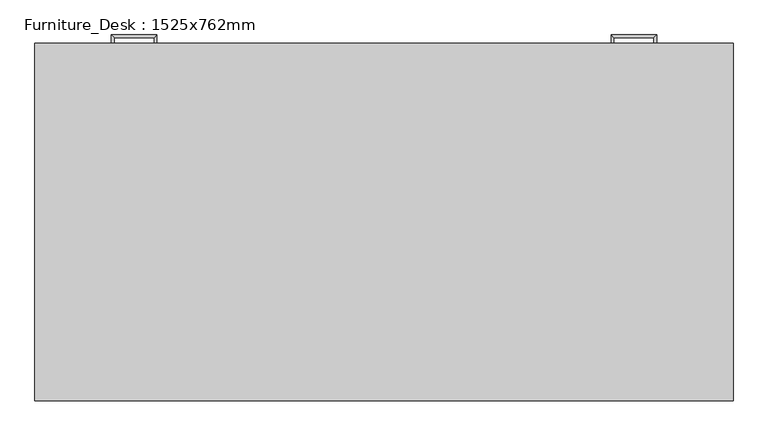
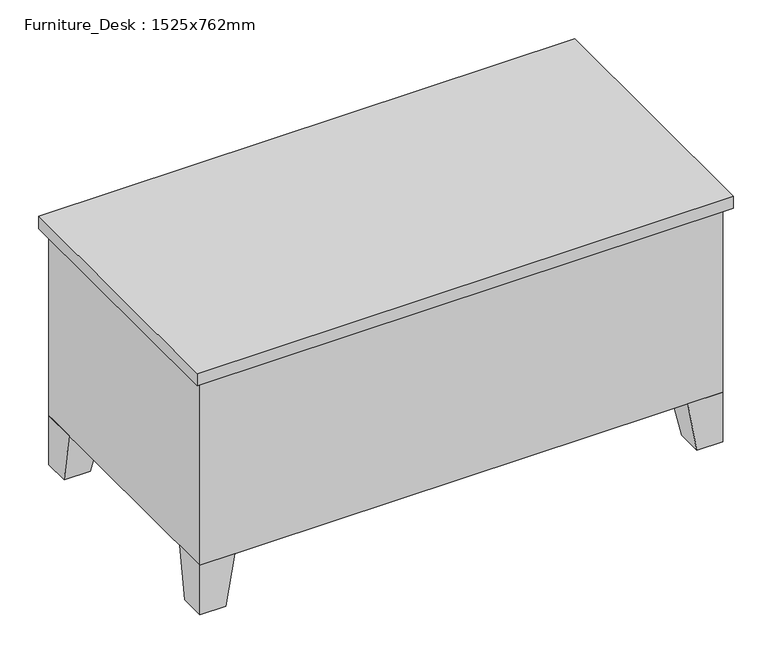
"""IFC4 building model written with IfcOpenShell, lengths in millimetres: furniture geometry, Furniture_Desk : 1525x762mm."""

import ifcopenshell
import ifcopenshell.guid

model = None  # the IFC model being written
_history = None  # IfcOwnerHistory: only IFC2X3 demands one
_inside = {}  # id of a spatial element -> (the spatial element, [elements in it])
_under = {}  # id of a project, library or spatial element -> (it, [spatial elements below it])
_declared = {}  # id of a project -> (the project, [libraries it declares])
_typed = {}  # id of a type object -> (the type object, [elements of that type])
_made_of = {}  # id of a material, layer set ... -> (it, [elements and type objects made of it])


def new_model(schema):
    """Start an empty IFC model of exactly this schema.

    Asked for "IFC4X3", IfcOpenShell would pick the latest addendum, in which some entities
    have other attributes; the version numbers below select the first issue.
    IFC2X3 requires an IfcOwnerHistory on every rooted entity: one is made here for all.
    """
    global model, _history
    if schema == "IFC4X3":
        model = ifcopenshell.file(schema_version=(4, 3, 0, 0))
    else:
        model = ifcopenshell.file(schema=schema)
    _inside.clear()
    _under.clear()
    _declared.clear()
    _typed.clear()
    _made_of.clear()
    _history = None
    if model.schema == "IFC2X3":
        org = make("IfcOrganization", Name="unknown")
        user = make(
            "IfcPersonAndOrganization",
            ThePerson=make("IfcPerson", FamilyName="unknown"),
            TheOrganization=org,
        )
        app = make(
            "IfcApplication",
            ApplicationDeveloper=org,
            Version="unknown",
            ApplicationFullName="unknown",
            ApplicationIdentifier="unknown",
        )
        _history = make(
            "IfcOwnerHistory",
            OwningUser=user,
            OwningApplication=app,
            ChangeAction="ADDED",
            CreationDate=0,
        )
    return model


def make(cls, **values):
    """One entity of the class cls with the attributes given. An attribute that is None is left unset."""
    return model.create_entity(
        cls, **{name: value for name, value in values.items() if value is not None}
    )


def rooted(cls, **values):
    """An entity with a GlobalId (a new one), such as an element, a storey or a relation."""
    return make(cls, GlobalId=ifcopenshell.guid.new(), OwnerHistory=_history, **values)


def si_unit(unit_type, name, prefix=None):
    """IfcSIUnit, for example si_unit("LENGTHUNIT", "METRE", prefix="MILLI")."""
    return make("IfcSIUnit", UnitType=unit_type, Prefix=prefix, Name=name)


def assignment(units):
    """IfcUnitAssignment: the units of a project."""
    return None if units is None else make("IfcUnitAssignment", Units=units)


def point(xyz):
    """IfcCartesianPoint."""
    return None if xyz is None else make("IfcCartesianPoint", Coordinates=xyz)


def direction(xyz):
    """IfcDirection."""
    return None if xyz is None else make("IfcDirection", DirectionRatios=xyz)


def frame(location, z_axis=None, x_axis=None):
    """IfcAxis2Placement3D, a coordinate frame: its origin and axes. An axis left out is left unset."""
    return make(
        "IfcAxis2Placement3D",
        Location=point(location),
        Axis=direction(z_axis),
        RefDirection=direction(x_axis),
    )


def origin():
    """The frame at (0, 0, 0) with its axes left unset."""
    return frame((0.0, 0.0, 0.0))


def place(relative_to, where):
    """IfcLocalPlacement: puts the frame where relative to a parent placement (None: the world)."""
    return make(
        "IfcLocalPlacement", PlacementRelTo=relative_to, RelativePlacement=where
    )


def context(
    kind, dimensions, precision=None, world=None, true_north=None, identifier=None
):
    """IfcGeometricRepresentationContext, for example the 3D "Model" context."""
    return make(
        "IfcGeometricRepresentationContext",
        ContextIdentifier=identifier,
        ContextType=kind,
        CoordinateSpaceDimension=dimensions,
        Precision=precision,
        WorldCoordinateSystem=world,
        TrueNorth=true_north,
    )


def project(units=None, contexts=None):
    """IfcProject with its units and contexts."""
    return rooted(
        "IfcProject",
        Name="project",
        RepresentationContexts=contexts,
        UnitsInContext=assignment(units),
    )


def spatial(cls, under=None, at=None, **own):
    """A site, building, storey or space (cls), placed at a placement, below another one or the project."""
    s = rooted(cls, ObjectPlacement=at, **own)
    if under is not None:
        _under.setdefault(under.id(), (under, []))[1].append(s)
    return s


def polyline(points):
    """IfcPolyline through the points."""
    return make("IfcPolyline", Points=[point(p) for p in points])


def outline(outer, holes=None, kind="AREA"):
    """IfcArbitraryClosedProfileDef: a profile drawn as a closed curve; with holes, ...WithVoids."""
    if holes is None:
        return make("IfcArbitraryClosedProfileDef", ProfileType=kind, OuterCurve=outer)
    return make(
        "IfcArbitraryProfileDefWithVoids",
        ProfileType=kind,
        OuterCurve=outer,
        InnerCurves=holes,
    )


def extrude(swept, where, along, depth):
    """IfcExtrudedAreaSolid: the profile swept, set in the frame where, extruded along a direction by depth."""
    return make(
        "IfcExtrudedAreaSolid",
        SweptArea=swept,
        Position=where,
        ExtrudedDirection=direction(along),
        Depth=depth,
    )


def faces_of(points, faces, orient=None, outer=None):
    """IfcFace entities. A face is a list of loops; a loop is a list of indices into points, from 0.

    orient and outer hold one flag for each loop. By default every Orientation is true, the
    first loop of a face is its IfcFaceOuterBound and the others are IfcFaceBound.
    """
    made = []
    for i, loops in enumerate(faces):
        bounds = []
        for j, loop in enumerate(loops):
            is_outer = j == 0 if outer is None else outer[i][j]
            bounds.append(
                make(
                    "IfcFaceOuterBound" if is_outer else "IfcFaceBound",
                    Bound=make("IfcPolyLoop", Polygon=[points[k] for k in loop]),
                    Orientation=True if orient is None else orient[i][j],
                )
            )
        made.append(make("IfcFace", Bounds=bounds))
    return made


def faceted_brep(points, faces, orient=None, outer=None, voids=None):
    """IfcFacetedBrep: a solid bounded by flat faces; with voids (closed shells), ...WithVoids."""
    shared = [point(p) for p in points]
    hull = make("IfcClosedShell", CfsFaces=faces_of(shared, faces, orient, outer))
    if voids is None:
        return make("IfcFacetedBrep", Outer=hull)
    return make(
        "IfcFacetedBrepWithVoids",
        Outer=hull,
        Voids=[
            make(cls, CfsFaces=faces_of(shared, fs, o, b)) for cls, fs, o, b in voids
        ],
    )


def shape(context_of_items, identifier, shape_type, items):
    """IfcShapeRepresentation: the items that make up one representation, for example the "Body"."""
    return make(
        "IfcShapeRepresentation",
        ContextOfItems=context_of_items,
        RepresentationIdentifier=identifier,
        RepresentationType=shape_type,
        Items=items,
    )


def source(mapping_origin, context_of_items, identifier, shape_type, items):
    """IfcRepresentationMap: a shape defined once, which mapped items show again and again."""
    return make(
        "IfcRepresentationMap",
        MappingOrigin=mapping_origin,
        MappedRepresentation=shape(context_of_items, identifier, shape_type, items),
    )


def transform(
    local_origin,
    x_axis=None,
    y_axis=None,
    z_axis=None,
    scale=None,
    scale2=None,
    scale3=None,
    uniform=True,
):
    """IfcCartesianTransformationOperator3D, or its non-uniform kind. x_axis, y_axis, z_axis: its Axis1, 2, 3."""
    if uniform:
        return make(
            "IfcCartesianTransformationOperator3D",
            Axis1=direction(x_axis),
            Axis2=direction(y_axis),
            LocalOrigin=point(local_origin),
            Scale=scale,
            Axis3=direction(z_axis),
        )
    return make(
        "IfcCartesianTransformationOperator3DnonUniform",
        Axis1=direction(x_axis),
        Axis2=direction(y_axis),
        LocalOrigin=point(local_origin),
        Scale=scale,
        Axis3=direction(z_axis),
        Scale2=scale2,
        Scale3=scale3,
    )


def mapped(mapping_source, mapping_target):
    """IfcMappedItem: shows the shape of a source again, moved by a transform."""
    return make(
        "IfcMappedItem", MappingSource=mapping_source, MappingTarget=mapping_target
    )


def made_of(thing, what):
    """Note that an element or type object is made of a material, layer set ...; save() writes the relation."""
    if what is not None:
        _made_of.setdefault(what.id(), (what, []))[1].append(thing)
    return thing


def element(
    cls,
    number,
    at=None,
    inside=None,
    cuts=None,
    type_object=None,
    material=None,
    context=None,
    identifier="Body",
    shape_type=None,
    held_by="IfcProductDefinitionShape",
    body=None,
    shapes=None,
    **own,
):
    """One element of the class cls, such as IfcWall. Its Tag is "e" and its number.

    at: its placement. inside: the storey or other place that contains it. cuts: it is an
    opening in that element (IfcRelVoidsElement). A single representation is given by context,
    identifier, shape_type and body (its items); several are given by shapes. held_by: the class
    of the entity that holds the representations. save() writes the other relations.
    """
    e = rooted(cls, Tag="e%d" % number, ObjectPlacement=at, **own)
    if body is not None:
        shapes = [shape(context, identifier, shape_type, body)]
    if shapes is not None:
        e.Representation = make(held_by, Representations=shapes)
    if inside is not None:
        _inside.setdefault(inside.id(), (inside, []))[1].append(e)
    if cuts is not None:
        rooted(
            "IfcRelVoidsElement", RelatingBuildingElement=cuts, RelatedOpeningElement=e
        )
    if type_object is not None:
        _typed.setdefault(type_object.id(), (type_object, []))[1].append(e)
    return made_of(e, material)


def aggregate(whole, parts):
    """IfcRelAggregates: a whole, such as a stair, and the parts it consists of."""
    return rooted("IfcRelAggregates", RelatingObject=whole, RelatedObjects=parts)


def save(model, path):
    """Write the relations noted so far, then the file.

    IfcRelAggregates (storeys below a building ...), IfcRelContainedInSpatialStructure (elements
    in a storey), IfcRelDefinesByType, IfcRelAssociatesMaterial and IfcRelDeclares: one each for
    every whole, place, type object, material and project.
    """
    for whole, parts in _under.values():
        aggregate(whole, parts)
    for where, things in _inside.values():
        rooted(
            "IfcRelContainedInSpatialStructure",
            RelatedElements=things,
            RelatingStructure=where,
        )
    for kind, things in _typed.values():
        rooted("IfcRelDefinesByType", RelatedObjects=things, RelatingType=kind)
    for what, things in _made_of.values():
        rooted("IfcRelAssociatesMaterial", RelatedObjects=things, RelatingMaterial=what)
    for by, libraries in _declared.values():
        rooted("IfcRelDeclares", RelatingContext=by, RelatedDefinitions=libraries)
    model.write(path)


def furniture_desk_1525x762mm_aed207d5(model_context):
    return source(origin(), model_context, "Body", "SolidModel", [
        extrude(outline(polyline([(1505.95, 762.0), (1137.65, 762.0), (1137.65, 774.7), (1505.95, 774.7), (1505.95, 762.0)])), frame((0.0, 0.0, 603.25), z_axis=(0.0, 0.0, 1.0), x_axis=(1.0, 0.0, 0.0)), (0.0, 0.0, 1.0), 101.6),
        extrude(outline(polyline([(1505.95, 762.0), (1137.65, 762.0), (1137.65, 774.7), (1505.95, 774.7), (1505.95, 762.0)])), frame((0.0, 0.0, 171.05), z_axis=(0.0, 0.0, 1.0), x_axis=(1.0, 0.0, 0.0)), (0.0, 0.0, 1.0), 413.15),
        extrude(outline(polyline([(387.35, 762.0), (19.05, 762.0), (19.05, 774.7), (387.35, 774.7), (387.35, 762.0)])), frame((0.0, 0.0, 602.85), z_axis=(0.0, 0.0, 1.0), x_axis=(1.0, 0.0, 0.0)), (0.0, 0.0, 1.0), 102.0),
        extrude(outline(polyline([(387.35, 762.0), (19.05, 762.0), (19.05, 774.7), (387.35, 774.7), (387.35, 762.0)])), frame((0.0, 0.0, 171.05), z_axis=(0.0, 0.0, 1.0), x_axis=(1.0, 0.0, 0.0)), (0.0, 0.0, 1.0), 171.45),
        extrude(outline(polyline([(387.35, 762.0), (19.05, 762.0), (19.05, 774.7), (387.35, 774.7), (387.35, 762.0)])), frame((0.0, 0.0, 482.2), z_axis=(0.0, 0.0, 1.0), x_axis=(1.0, 0.0, 0.0)), (0.0, 0.0, 1.0), 101.6),
        extrude(outline(polyline([(387.35, 762.0), (19.05, 762.0), (19.05, 774.7), (387.35, 774.7), (387.35, 762.0)])), frame((0.0, 0.0, 361.55), z_axis=(0.0, 0.0, 1.0), x_axis=(1.0, 0.0, 0.0)), (0.0, 0.0, 1.0), 101.6),
        faceted_brep([(1423.4, 762.0, 152.0), (1423.4, 660.4, 152.0), (1525.0, 660.4, 152.0), (1525.0, 762.0, 152.0), (1448.8, 762.0, 0.0), (1525.0, 762.0, 0.0), (1525.0, 685.8, 0.0), (1448.8, 685.8, 0.0)], [[[0, 1, 2, 3]], [[4, 5, 6, 7]], [[4, 7, 1, 0]], [[7, 6, 2, 1]], [[6, 5, 3, 2]], [[5, 4, 0, 3]]]),
        faceted_brep([(1423.4, 0.0, 152.0), (1525.0, 0.0, 152.0), (1525.0, 101.6, 152.0), (1423.4, 101.6, 152.0), (1448.8, 0.0, 0.0), (1448.8, 76.2, 0.0), (1525.0, 76.2, 0.0), (1525.0, 0.0, 0.0)], [[[0, 1, 2, 3]], [[4, 5, 6, 7]], [[4, 7, 1, 0]], [[7, 6, 2, 1]], [[6, 5, 3, 2]], [[5, 4, 0, 3]]]),
        faceted_brep([(101.6, 0.0, 152.0), (101.6, 101.6, 152.0), (0.0, 101.6, 152.0), (0.0, 0.0, 152.0), (76.2, 0.0, 0.0), (0.0, 0.0, 0.0), (0.0, 76.2, 0.0), (76.2, 76.2, 0.0)], [[[0, 1, 2, 3]], [[4, 5, 6, 7]], [[4, 7, 1, 0]], [[7, 6, 2, 1]], [[6, 5, 3, 2]], [[5, 4, 0, 3]]]),
        faceted_brep([(101.6, 762.0, 152.0), (0.0, 762.0, 152.0), (0.0, 660.4, 152.0), (101.6, 660.4, 152.0), (76.2, 762.0, 0.0), (76.2, 685.8, 0.0), (0.0, 685.8, 0.0), (0.0, 762.0, 0.0)], [[[0, 1, 2, 3]], [[4, 5, 6, 7]], [[4, 7, 1, 0]], [[7, 6, 2, 1]], [[6, 5, 3, 2]], [[5, 4, 0, 3]]]),
        extrude(outline(polyline([(1544.05, 781.05), (1544.05, -19.05), (-19.05, -19.05), (-19.05, 781.05), (1544.05, 781.05)])), frame((0.0, 0.0, 723.9), z_axis=(0.0, 0.0, 1.0), x_axis=(1.0, 0.0, 0.0)), (0.0, 0.0, 1.0), 38.1),
        extrude(outline(polyline([(406.4, 762.0), (406.4, 50.8), (1118.6, 50.8), (1118.6, 762.0), (1525.0, 762.0), (1525.0, 0.0), (0.0, 0.0), (0.0, 762.0), (406.4, 762.0)])), frame((0.0, 0.0, 152.0), z_axis=(0.0, 0.0, 1.0), x_axis=(1.0, 0.0, 0.0)), (0.0, 0.0, 1.0), 571.9),
        faceted_brep([(1366.25, 774.7, 546.1), (1366.25, 774.7, 533.4), (1372.6, 774.7, 533.4), (1372.6, 774.7, 546.1), (1366.25, 793.75, 546.1), (1366.25, 793.75, 533.4), (1372.6, 800.1, 533.4), (1372.6, 800.1, 546.1), (1277.35, 793.75, 546.1), (1277.35, 793.75, 533.4), (1271.0, 800.1, 533.4), (1271.0, 800.1, 546.1), (1277.35, 774.7, 546.1), (1271.0, 774.7, 546.1), (1271.0, 774.7, 533.4), (1277.35, 774.7, 533.4)], [[[0, 1, 2, 3]], [[1, 0, 4, 5]], [[2, 1, 5, 6]], [[3, 2, 6, 7]], [[0, 3, 7, 4]], [[5, 4, 8, 9]], [[6, 5, 9, 10]], [[7, 6, 10, 11]], [[4, 7, 11, 8]], [[12, 13, 14, 15]], [[9, 8, 12, 15]], [[10, 9, 15, 14]], [[11, 10, 14, 13]], [[8, 11, 13, 12]]]),
        faceted_brep([(1366.25, 774.7, 666.75), (1366.25, 774.7, 654.05), (1372.6, 774.7, 654.05), (1372.6, 774.7, 666.75), (1366.25, 793.75, 666.75), (1366.25, 793.75, 654.05), (1372.6, 800.1, 654.05), (1372.6, 800.1, 666.75), (1277.35, 793.75, 666.75), (1277.35, 793.75, 654.05), (1271.0, 800.1, 654.05), (1271.0, 800.1, 666.75), (1277.35, 774.7, 666.75), (1271.0, 774.7, 666.75), (1271.0, 774.7, 654.05), (1277.35, 774.7, 654.05)], [[[0, 1, 2, 3]], [[1, 0, 4, 5]], [[2, 1, 5, 6]], [[3, 2, 6, 7]], [[0, 3, 7, 4]], [[5, 4, 8, 9]], [[6, 5, 9, 10]], [[7, 6, 10, 11]], [[4, 7, 11, 8]], [[12, 13, 14, 15]], [[9, 8, 12, 15]], [[10, 9, 15, 14]], [[11, 10, 14, 13]], [[8, 11, 13, 12]]]),
        faceted_brep([(158.75, 774.7, 304.8), (152.4, 774.7, 304.8), (152.4, 774.7, 292.1), (158.75, 774.7, 292.1), (158.75, 793.75, 304.8), (152.4, 800.1, 304.8), (152.4, 800.1, 292.1), (158.75, 793.75, 292.1), (247.65, 793.75, 304.8), (254.0, 800.1, 304.8), (254.0, 800.1, 292.1), (247.65, 793.75, 292.1), (247.65, 774.7, 304.8), (247.65, 774.7, 292.1), (254.0, 774.7, 292.1), (254.0, 774.7, 304.8)], [[[0, 1, 2, 3]], [[1, 0, 4, 5]], [[2, 1, 5, 6]], [[3, 2, 6, 7]], [[0, 3, 7, 4]], [[5, 4, 8, 9]], [[6, 5, 9, 10]], [[7, 6, 10, 11]], [[4, 7, 11, 8]], [[12, 13, 14, 15]], [[9, 8, 12, 15]], [[10, 9, 15, 14]], [[11, 10, 14, 13]], [[8, 11, 13, 12]]]),
        faceted_brep([(158.75, 774.7, 425.45), (152.4, 774.7, 425.45), (152.4, 774.7, 412.75), (158.75, 774.7, 412.75), (158.75, 793.75, 425.45), (152.4, 800.1, 425.45), (152.4, 800.1, 412.75), (158.75, 793.75, 412.75), (247.65, 793.75, 425.45), (254.0, 800.1, 425.45), (254.0, 800.1, 412.75), (247.65, 793.75, 412.75), (247.65, 774.7, 425.45), (247.65, 774.7, 412.75), (254.0, 774.7, 412.75), (254.0, 774.7, 425.45)], [[[0, 1, 2, 3]], [[1, 0, 4, 5]], [[2, 1, 5, 6]], [[3, 2, 6, 7]], [[0, 3, 7, 4]], [[5, 4, 8, 9]], [[6, 5, 9, 10]], [[7, 6, 10, 11]], [[4, 7, 11, 8]], [[12, 13, 14, 15]], [[9, 8, 12, 15]], [[10, 9, 15, 14]], [[11, 10, 14, 13]], [[8, 11, 13, 12]]]),
        faceted_brep([(158.75, 774.7, 546.1), (152.4, 774.7, 546.1), (152.4, 774.7, 533.4), (158.75, 774.7, 533.4), (158.75, 793.75, 546.1), (152.4, 800.1, 546.1), (152.4, 800.1, 533.4), (158.75, 793.75, 533.4), (247.65, 793.75, 546.1), (254.0, 800.1, 546.1), (254.0, 800.1, 533.4), (247.65, 793.75, 533.4), (247.65, 774.7, 546.1), (247.65, 774.7, 533.4), (254.0, 774.7, 533.4), (254.0, 774.7, 546.1)], [[[0, 1, 2, 3]], [[1, 0, 4, 5]], [[2, 1, 5, 6]], [[3, 2, 6, 7]], [[0, 3, 7, 4]], [[5, 4, 8, 9]], [[6, 5, 9, 10]], [[7, 6, 10, 11]], [[4, 7, 11, 8]], [[12, 13, 14, 15]], [[9, 8, 12, 15]], [[10, 9, 15, 14]], [[11, 10, 14, 13]], [[8, 11, 13, 12]]]),
        faceted_brep([(158.75, 774.7, 666.75), (152.4, 774.7, 666.75), (152.4, 774.7, 654.05), (158.75, 774.7, 654.05), (158.75, 793.75, 666.75), (152.4, 800.1, 666.75), (152.4, 800.1, 654.05), (158.75, 793.75, 654.05), (247.65, 793.75, 666.75), (254.0, 800.1, 666.75), (254.0, 800.1, 654.05), (247.65, 793.75, 654.05), (247.65, 774.7, 666.75), (247.65, 774.7, 654.05), (254.0, 774.7, 654.05), (254.0, 774.7, 666.75)], [[[0, 1, 2, 3]], [[1, 0, 4, 5]], [[2, 1, 5, 6]], [[3, 2, 6, 7]], [[0, 3, 7, 4]], [[5, 4, 8, 9]], [[6, 5, 9, 10]], [[7, 6, 10, 11]], [[4, 7, 11, 8]], [[12, 13, 14, 15]], [[9, 8, 12, 15]], [[10, 9, 15, 14]], [[11, 10, 14, 13]], [[8, 11, 13, 12]]]),
    ])


if __name__ == "__main__":
    model = new_model("IFC4")
    model_context = context("Model", 3, world=origin())
    ifc_project = project(units=[si_unit("LENGTHUNIT", "METRE", prefix="MILLI")], contexts=[model_context])
    site = spatial("IfcSite", under=ifc_project)
    building = spatial("IfcBuilding", under=site)
    placement = place(None, origin())
    furniture_desk_1525x762mm_shape = furniture_desk_1525x762mm_aed207d5(model_context)
    element("IfcFurniture", 1, ObjectType="Furniture_Desk : 1525x762mm", at=placement, inside=building, context=model_context, shape_type="MappedRepresentation", body=[
        mapped(furniture_desk_1525x762mm_shape, transform((0.0, 0.0, 0.0), x_axis=(1.0, 0.0, 0.0), y_axis=(0.0, 1.0, 0.0), z_axis=(0.0, 0.0, 1.0))),
    ])
    save(model, "model.ifc")

# Revit data of these elements
# Type "Furniture_Desk : 1525x762mm"
#   Keynote = "N"
#   Width = 1525 mm
#   Leg Height = 152 mm
#   Height = 762 mm
#   Depth = 762 mm
#   Top Material = Cherry
#   Handle/Leg Material = Steel, Chrome Plated
#   Body Material = Laminate, Ivory, Matte
#   Default Elevation = 0
#   Assembly Code = ""
# Element 1 (IfcFurniture, "Furniture_Desk : 1525x762mm")
#   Materials on its faces: "Steel, Chrome Plated", "Laminate, Ivory, Matte", "Cherry"
# Materials
#   "Cherry": class "Wood", colour RGB 226 177 128, transparency 0, Description = "Prunus Serotina", Cost = 0
#   "Steel, Chrome Plated": class "Metal", colour RGB 216 216 216, transparency 0, Description = "Chromiuim plated steel", Cost = 0
#   "Laminate, Ivory, Matte": class "Plastic", colour RGB 247 247 239, transparency 0, Description = "Plastic Laminate - Ivory, Matte", Cost = 0
